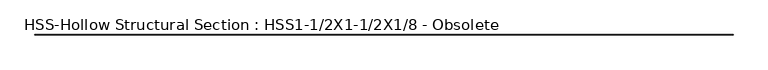
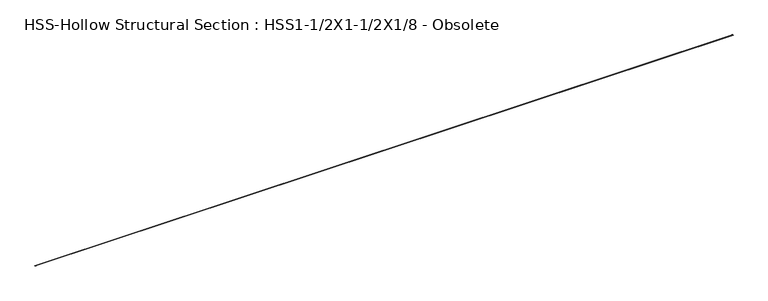
"""IFC4 building model written with IfcOpenShell, lengths in millimetres: beam geometry, HSS-Hollow Structural Section : HSS1-1/2X1-1/2X1/8 - Obsolete."""

from ifc_helpers import new_model, si_unit, point, frame, frame_2d, origin, place, context, project, spatial, polyline, circle_curve, trimmed, segment, composite_curve, outline, extrude, source, transform, mapped, element, save


def hss_hollow_structural_section_hss1_1_2x1_1_2x1_8_obsolete_b8429d67(model_context):
    return source(origin(), model_context, "Body", "SweptSolid", [
        extrude(outline(composite_curve([segment(polyline([(19.05, 13.1572), (19.05, -13.1572)]), True, "CONTINUOUS"), segment(trimmed(circle_curve(frame_2d((13.1572, -13.1572)), 5.8928), [point((19.05, -13.1572))], [point((13.1572, -19.05))], False, "CARTESIAN"), True, "CONTINUOUS"), segment(polyline([(13.1572, -19.05), (-13.1572, -19.05)]), True, "CONTINUOUS"), segment(trimmed(circle_curve(frame_2d((-13.1572, -13.1572)), 5.8928), [point((-13.1572, -19.05))], [point((-19.05, -13.1572))], False, "CARTESIAN"), True, "CONTINUOUS"), segment(polyline([(-19.05, -13.1572), (-19.05, 13.1572)]), True, "CONTINUOUS"), segment(trimmed(circle_curve(frame_2d((-13.1572, 13.1572)), 5.8928), [point((-19.05, 13.1572))], [point((-13.1572, 19.05))], False, "CARTESIAN"), True, "CONTINUOUS"), segment(polyline([(-13.1572, 19.05), (13.1572, 19.05)]), True, "CONTINUOUS"), segment(trimmed(circle_curve(frame_2d((13.1572, 13.1572)), 5.8928), [point((13.1572, 19.05))], [point((19.05, 13.1572))], False, "CARTESIAN"), True, "CONTINUOUS")], self_intersect=False), holes=[composite_curve([segment(trimmed(circle_curve(frame_2d((-13.1572, 13.1572)), 2.9464), [point((-13.1572, 16.1036))], [point((-16.1036, 13.1572))], True, "CARTESIAN"), True, "CONTINUOUS"), segment(polyline([(-16.1036, 13.1572), (-16.1036, -13.1572)]), True, "CONTINUOUS"), segment(trimmed(circle_curve(frame_2d((-13.1572, -13.1572)), 2.9464), [point((-16.1036, -13.1572))], [point((-13.1572, -16.1036))], True, "CARTESIAN"), True, "CONTINUOUS"), segment(polyline([(-13.1572, -16.1036), (13.1572, -16.1036)]), True, "CONTINUOUS"), segment(trimmed(circle_curve(frame_2d((13.1572, -13.1572)), 2.9464), [point((13.1572, -16.1036))], [point((16.1036, -13.1572))], True, "CARTESIAN"), True, "CONTINUOUS"), segment(polyline([(16.1036, -13.1572), (16.1036, 13.1572)]), True, "CONTINUOUS"), segment(trimmed(circle_curve(frame_2d((13.1572, 13.1572)), 2.9464), [point((16.1036, 13.1572))], [point((13.1572, 16.1036))], True, "CARTESIAN"), True, "CONTINUOUS"), segment(polyline([(13.1572, 16.1036), (-13.1572, 16.1036)]), True, "CONTINUOUS")], self_intersect=False)]), frame((-44535.7377, 0.0, 0.0), z_axis=(1.0, 0.0, 0.0), x_axis=(0.0, 1.0, 0.0)), (0.0, 0.0, 1.0), 89071.4754),
    ])


if __name__ == "__main__":
    model = new_model("IFC4")
    model_context = context("Model", 3, world=origin())
    ifc_project = project(units=[si_unit("LENGTHUNIT", "METRE", prefix="MILLI")], contexts=[model_context])
    site = spatial("IfcSite", under=ifc_project)
    building = spatial("IfcBuilding", under=site)
    placement = place(None, origin())
    hss_hollow_structural_section_hss1_1_2x1_1_2x1_8_obsolete_shape = hss_hollow_structural_section_hss1_1_2x1_1_2x1_8_obsolete_b8429d67(model_context)
    element("IfcBeam", 1, ObjectType="HSS-Hollow Structural Section : HSS1-1/2X1-1/2X1/8 - Obsolete", at=placement, inside=building, context=model_context, shape_type="MappedRepresentation", body=[
        mapped(hss_hollow_structural_section_hss1_1_2x1_1_2x1_8_obsolete_shape, transform((0.0, 0.0, 0.0), x_axis=(1.0, 0.0, 0.0), y_axis=(0.0, 1.0, 0.0), z_axis=(0.0, 0.0, 1.0))),
    ])
    save(model, "model.ifc")

# Revit data of these elements
# Type "HSS-Hollow Structural Section : HSS1-1/2X1-1/2X1/8 - Obsolete"
#   Assembly Code = "B10"
#   Shape = "Square"
#   W = 2.19
#   Ht = 0' - 1 1/2"
#   Length [instance default] = 5' - 0"
#   b = 0' - 1 1/2"
#   kr = 0' - 0.232"
#   t = 0' - 0.116"
#   A = 0.00423611 SF
#   Structural Material [instance default] = 1 1/2" X 1 1/2" x 1/8" ALUM. TUBE
# Element 1 (IfcBeam, "HSS-Hollow Structural Section : HSS1-1/2X1-1/2X1/8 - Obsolete")
#   Materials on its faces: "1 1/2\" X 1 1/2\" x 1/8\" ALUM. TUBE"
# Materials
#   "1 1/2\" X 1 1/2\" x 1/8\" ALUM. TUBE": class "Metal", colour RGB 199 199 199, transparency 0, Description = "Carbon steel", Cost = 0
